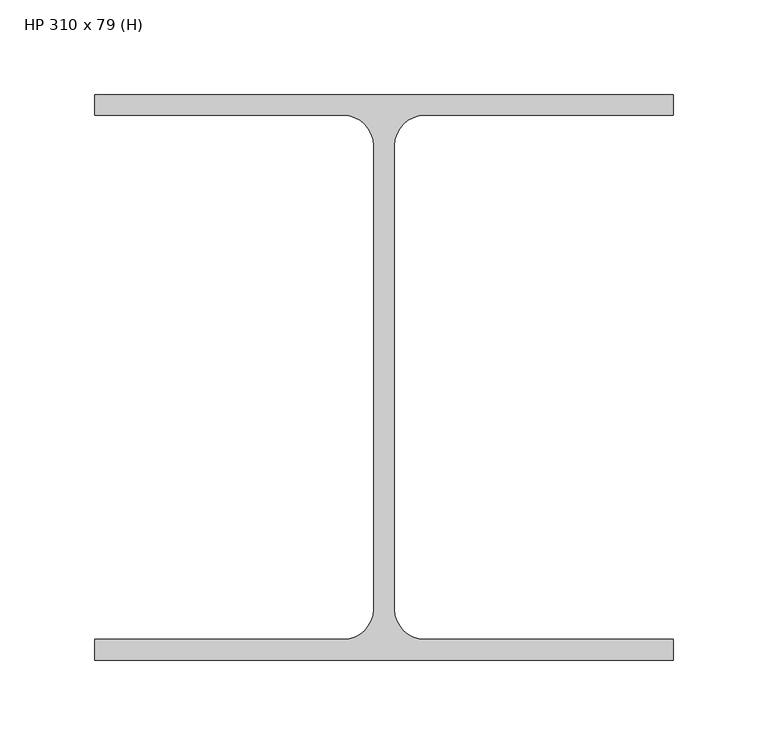
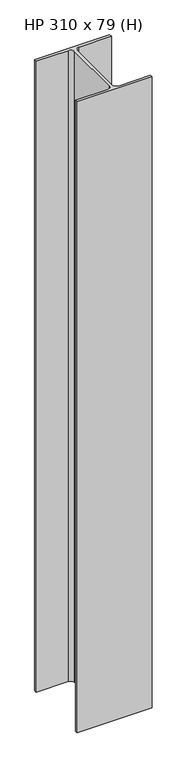
"""IFC4 building model written with IfcOpenShell, lengths in millimetres: column geometry, Pilar de Aço - H : HP 310 x 79 (H)."""

from ifc_helpers import new_model, si_unit, point, frame_2d, origin, origin_with_axes, place, context, project, spatial, polyline, circle_curve, trimmed, segment, composite_curve, outline, extrude, source, transform, mapped, element, save


def hp_310_x_79_h_687425f2(model_context):
    return source(origin(), model_context, "Body", "SweptSolid", [
        extrude(outline(composite_curve([segment(polyline([(153.0, 149.5), (153.0, 138.5), (21.5, 138.5)]), True, "CONTINUOUS"), segment(trimmed(circle_curve(frame_2d((21.5, 122.5)), 16.0), [point((21.5, 138.5))], [point((5.5, 122.5))], True, "CARTESIAN"), True, "CONTINUOUS"), segment(polyline([(5.5, 122.5), (5.5, -122.5)]), True, "CONTINUOUS"), segment(trimmed(circle_curve(frame_2d((21.5, -122.5)), 16.0), [point((5.5, -122.5))], [point((21.5, -138.5))], True, "CARTESIAN"), True, "CONTINUOUS"), segment(polyline([(21.5, -138.5), (153.0, -138.5), (153.0, -149.5), (-153.0, -149.5), (-153.0, -138.5), (-21.5, -138.5)]), True, "CONTINUOUS"), segment(trimmed(circle_curve(frame_2d((-21.5, -122.5)), 16.0), [point((-21.5, -138.5))], [point((-5.5, -122.5))], True, "CARTESIAN"), True, "CONTINUOUS"), segment(polyline([(-5.5, -122.5), (-5.5, 122.5)]), True, "CONTINUOUS"), segment(trimmed(circle_curve(frame_2d((-21.5, 122.5)), 16.0), [point((-5.5, 122.5))], [point((-21.5, 138.5))], True, "CARTESIAN"), True, "CONTINUOUS"), segment(polyline([(-21.5, 138.5), (-153.0, 138.5), (-153.0, 149.5), (153.0, 149.5)]), True, "CONTINUOUS")], self_intersect=False)), origin_with_axes(), (0.0, 0.0, 1.0), 2720.0),
    ])


if __name__ == "__main__":
    model = new_model("IFC4")
    model_context = context("Model", 3, world=origin())
    ifc_project = project(units=[si_unit("LENGTHUNIT", "METRE", prefix="MILLI")], contexts=[model_context])
    site = spatial("IfcSite", under=ifc_project)
    building = spatial("IfcBuilding", under=site)
    placement = place(None, origin())
    hp_310_x_79_h_shape = hp_310_x_79_h_687425f2(model_context)
    element("IfcColumn", 1, ObjectType="Pilar de Aço - H : HP 310 x 79 (H)", at=placement, inside=building, context=model_context, shape_type="MappedRepresentation", body=[
        mapped(hp_310_x_79_h_shape, transform((0.0, 0.0, 0.0), x_axis=(1.0, 0.0, 0.0), y_axis=(0.0, 1.0, 0.0), z_axis=(0.0, 0.0, 1.0))),
    ])
    save(model, "model.ifc")

# Revit data of these elements
# Type "Pilar de Aço - H : HP 310 x 79 (H)"
#   SINAPI = ""
#   Área da seção = 100 m²
#   tw = 1.10 cm
#   tf = 1.10 cm
#   h = 27.70 cm
#   d' = 24.50 cm
#   d = 29.90 cm
#   bf = 30.60 cm
#   R = 1.60 cm
#   Massa Linear kg/m = 79
#   Aço = Metal - Aço 345MPa
#   Assembly Code = ""
# Materials
#   "Metal - Aço 345MPa": class "Metal", colour RGB 189 187 185, transparency 0, Cost = 0
